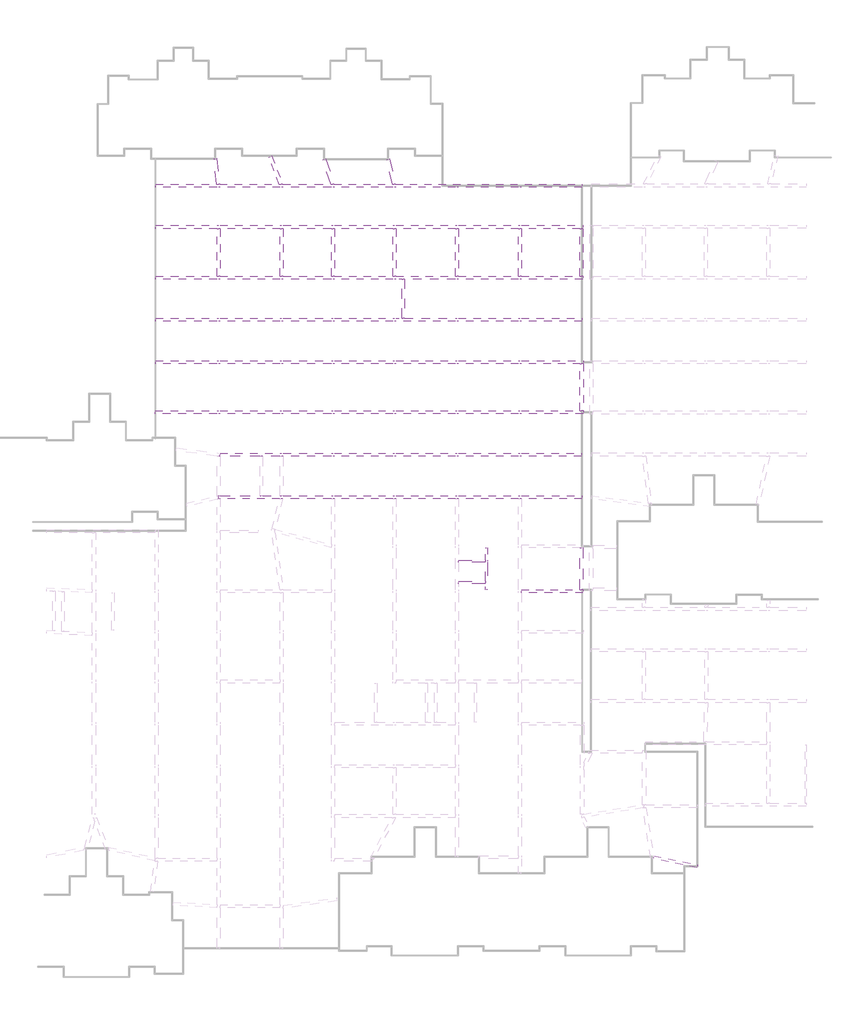
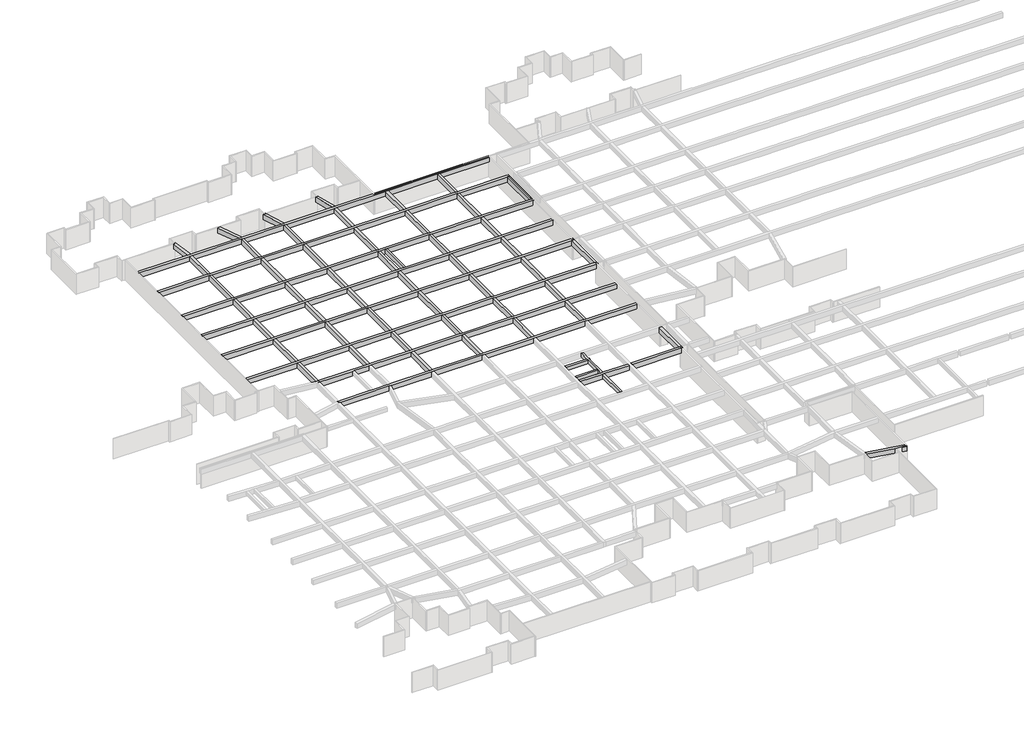
# One storey, part 11 of 16: 27 beams.
"""IFC4 building model written with IfcOpenShell, lengths in millimetres."""

from ifc_helpers import new_model, si_unit, frame, origin, place, context, project, spatial, polyline, outline, extrude, faceted_brep, element, save

model = new_model("IFC4")

# Units and contexts
model_context = context("Model", 3, world=origin())
ifc_project = project(units=[si_unit("LENGTHUNIT", "METRE", prefix="MILLI")], contexts=[model_context])

# Site, building, storey
site = spatial("IfcSite", under=ifc_project)
building = spatial("IfcBuilding", under=site)
storey = spatial("IfcBuildingStorey", under=building, Name="户型图", Elevation=0.0)

# Beams
placement = place(None, origin())
element("IfcBeam", 1, ObjectType="混凝土 - 矩形梁 : KL_beam", at=placement, inside=storey, context=model_context, shape_type="Brep", body=[
    faceted_brep([(255003.757676, -132325.7214763, 3300.0), (255003.757676, -132725.7214763, 3300.0), (255003.757676, -132725.7214763, 2500.0), (255003.757676, -132325.7214763, 2500.0), (200203.757676, -132325.7214763, 3300.0), (200203.757676, -132325.7214763, 2500.0), (200203.757676, -132725.7214763, 2500.0), (200203.757676, -132725.7214763, 3300.0), (231074.340029, -132325.7214763, 3300.0), (230661.8664477, -132325.7214763, 3300.0), (223163.2360526, -132325.7214763, 3300.0), (222740.8165445, -132325.7214763, 3300.0), (216536.3465944, -132325.7214763, 3300.0), (216107.8885969, -132325.7214763, 3300.0), (208493.8825468, -132325.7214763, 3300.0), (208090.4250487, -132325.7214763, 3300.0), (208121.0257524, -132725.7214763, 3300.0), (208521.0257524, -132725.7214763, 3300.0), (216198.8904026, -132725.7214763, 3300.0), (216598.8904026, -132725.7214763, 3300.0), (222798.8904026, -132725.7214763, 3300.0), (223198.8904026, -132725.7214763, 3300.0), (230718.438254, -132725.7214763, 3300.0), (231118.438254, -132725.7214763, 3300.0), (238718.438254, -132725.7214763, 3300.0), (239118.438254, -132725.7214763, 3300.0), (246818.438254, -132725.7214763, 3300.0), (247218.438254, -132725.7214763, 3300.0), (208121.0257524, -132725.7214763, 2500.0), (208521.0257524, -132725.7214763, 2500.0), (216198.8904026, -132725.7214763, 2500.0), (216598.8904026, -132725.7214763, 2500.0), (222798.8904026, -132725.7214763, 2500.0), (223198.8904026, -132725.7214763, 2500.0), (230718.438254, -132725.7214763, 2500.0), (231118.438254, -132725.7214763, 2500.0), (238718.438254, -132725.7214763, 2500.0), (239118.438254, -132725.7214763, 2500.0), (246818.438254, -132725.7214763, 2500.0), (247218.438254, -132725.7214763, 2500.0), (208090.4250487, -132325.7214763, 2500.0), (208493.8825468, -132325.7214763, 2500.0), (216107.8885969, -132325.7214763, 2500.0), (216536.3465944, -132325.7214763, 2500.0), (222740.8165445, -132325.7214763, 2500.0), (223163.2360526, -132325.7214763, 2500.0), (230661.8664477, -132325.7214763, 2500.0), (231074.340029, -132325.7214763, 2500.0)], [[[0, 1, 2, 3]], [[4, 5, 6, 7]], [[1, 0, 8, 9, 10, 11, 12, 13, 14, 15, 4, 7, 16, 17, 18, 19, 20, 21, 22, 23, 24, 25, 26, 27]], [[2, 1, 27, 26, 25, 24, 23, 22, 21, 20, 19, 18, 17, 16, 7, 6, 28, 29, 30, 31, 32, 33, 34, 35, 36, 37, 38, 39]], [[3, 2, 39, 38, 37, 36, 35, 34, 33, 32, 31, 30, 29, 28, 6, 5, 40, 41, 42, 43, 44, 45, 46, 47]], [[0, 3, 47, 46, 45, 44, 43, 42, 41, 40, 5, 4, 15, 14, 13, 12, 11, 10, 9, 8]]]),
])
element("IfcBeam", 2, ObjectType="混凝土 - 矩形梁 : KL_beam", at=placement, inside=storey, context=model_context, shape_type="SweptSolid", body=[
    extrude(outline(polyline([(207660.2352637, -129060.9134022), (208056.8073952, -129008.6587899), (208493.8825468, -132325.7214763), (208090.4250487, -132325.7214763), (207660.2352637, -129060.9134022)])), frame((0.0, 0.0, 2500.0), z_axis=(0.0, 0.0, 1.0), x_axis=(1.0, 0.0, 0.0)), (0.0, 0.0, 1.0), 800.0),
])
element("IfcBeam", 3, ObjectType="混凝土 - 矩形梁 : KL_beam", at=placement, inside=storey, context=model_context, shape_type="SweptSolid", body=[
    extrude(outline(polyline([(214772.1689398, -128846.0528041), (215145.6011104, -128702.7056243), (216536.3465944, -132325.7214763), (216107.8885969, -132325.7214763), (214772.1689398, -128846.0528041)])), frame((0.0, 0.0, 2500.0), z_axis=(0.0, 0.0, 1.0), x_axis=(1.0, 0.0, 0.0)), (0.0, 0.0, 1.0), 800.0),
])
element("IfcBeam", 4, ObjectType="混凝土 - 矩形梁 : KL_beam", at=placement, inside=storey, context=model_context, shape_type="SweptSolid", body=[
    extrude(outline(polyline([(221670.6359164, -129173.2052189), (222049.406302, -129044.6245246), (223163.2360526, -132325.7214763), (222740.8165445, -132325.7214763), (221670.6359164, -129173.2052189)])), frame((0.0, 0.0, 2500.0), z_axis=(0.0, 0.0, 1.0), x_axis=(1.0, 0.0, 0.0)), (0.0, 0.0, 1.0), 800.0),
])
element("IfcBeam", 5, ObjectType="混凝土 - 矩形梁 : KL_beam", at=placement, inside=storey, context=model_context, shape_type="SweptSolid", body=[
    extrude(outline(polyline([(229864.5673641, -129157.7515328), (230252.4709955, -129060.125856), (231074.340029, -132325.7214763), (230661.8664477, -132325.7214763), (229864.5673641, -129157.7515328)])), frame((0.0, 0.0, 2500.0), z_axis=(0.0, 0.0, 1.0), x_axis=(1.0, 0.0, 0.0)), (0.0, 0.0, 1.0), 800.0),
])
element("IfcBeam", 6, ObjectType="混凝土 - 矩形梁 : KL_beam", at=placement, inside=storey, context=model_context, shape_type="Brep", body=[
    faceted_brep([(200203.757676, -137625.7214763, 3300.0), (200203.757676, -137625.7214763, 2500.0), (200203.757676, -138025.7214763, 2500.0), (200203.757676, -138025.7214763, 3300.0), (208121.0257524, -138025.7214763, 3300.0), (208521.0257524, -138025.7214763, 3300.0), (216198.8904026, -138025.7214763, 3300.0), (216598.8904026, -138025.7214763, 3300.0), (222798.8904026, -138025.7214763, 3300.0), (223198.8904026, -138025.7214763, 3300.0), (230718.438254, -138025.7214763, 3300.0), (231118.438254, -138025.7214763, 3300.0), (238718.438254, -138025.7214763, 3300.0), (239118.438254, -138025.7214763, 3300.0), (246818.438254, -138025.7214763, 3300.0), (247218.438254, -138025.7214763, 3300.0), (254703.757676, -138025.7214763, 3300.0), (255103.757676, -138025.7214763, 3300.0), (255103.757676, -137625.7214763, 3300.0), (247218.438254, -137625.7214763, 3300.0), (246818.438254, -137625.7214763, 3300.0), (239118.438254, -137625.7214763, 3300.0), (238718.438254, -137625.7214763, 3300.0), (231118.438254, -137625.7214763, 3300.0), (230718.438254, -137625.7214763, 3300.0), (223198.8904026, -137625.7214763, 3300.0), (222798.8904026, -137625.7214763, 3300.0), (216598.8904026, -137625.7214763, 3300.0), (216198.8904026, -137625.7214763, 3300.0), (208521.0257524, -137625.7214763, 3300.0), (208121.0257524, -137625.7214763, 3300.0), (208121.0257524, -138025.7214763, 2500.0), (208521.0257524, -138025.7214763, 2500.0), (216198.8904026, -138025.7214763, 2500.0), (216598.8904026, -138025.7214763, 2500.0), (222798.8904026, -138025.7214763, 2500.0), (223198.8904026, -138025.7214763, 2500.0), (230718.438254, -138025.7214763, 2500.0), (231118.438254, -138025.7214763, 2500.0), (238718.438254, -138025.7214763, 2500.0), (239118.438254, -138025.7214763, 2500.0), (246818.438254, -138025.7214763, 2500.0), (247218.438254, -138025.7214763, 2500.0), (254703.757676, -138025.7214763, 2500.0), (255103.757676, -138025.7214763, 2500.0), (208121.0257524, -137625.7214763, 2500.0), (208521.0257524, -137625.7214763, 2500.0), (216198.8904026, -137625.7214763, 2500.0), (216598.8904026, -137625.7214763, 2500.0), (222798.8904026, -137625.7214763, 2500.0), (223198.8904026, -137625.7214763, 2500.0), (230718.438254, -137625.7214763, 2500.0), (231118.438254, -137625.7214763, 2500.0), (238718.438254, -137625.7214763, 2500.0), (239118.438254, -137625.7214763, 2500.0), (246818.438254, -137625.7214763, 2500.0), (247218.438254, -137625.7214763, 2500.0), (255103.757676, -137625.7214763, 2500.0)], [[[0, 1, 2, 3]], [[0, 3, 4, 5, 6, 7, 8, 9, 10, 11, 12, 13, 14, 15, 16, 17, 18, 19, 20, 21, 22, 23, 24, 25, 26, 27, 28, 29, 30]], [[3, 2, 31, 32, 33, 34, 35, 36, 37, 38, 39, 40, 41, 42, 43, 44, 17, 16, 15, 14, 13, 12, 11, 10, 9, 8, 7, 6, 5, 4]], [[2, 1, 45, 46, 47, 48, 49, 50, 51, 52, 53, 54, 55, 56, 57, 44, 43, 42, 41, 40, 39, 38, 37, 36, 35, 34, 33, 32, 31]], [[1, 0, 30, 29, 28, 27, 26, 25, 24, 23, 22, 21, 20, 19, 18, 57, 56, 55, 54, 53, 52, 51, 50, 49, 48, 47, 46, 45]], [[18, 17, 44, 57]]]),
])
element("IfcBeam", 7, ObjectType="混凝土 - 矩形梁 : KL_beam", at=placement, inside=storey, context=model_context, shape_type="Brep", body=[
    faceted_brep([(200203.757676, -144125.7214763, 3300.0), (200203.757676, -144125.7214763, 2500.0), (200203.757676, -144525.7214763, 2500.0), (200203.757676, -144525.7214763, 3300.0), (208121.0257524, -144525.7214763, 3300.0), (208521.0257524, -144525.7214763, 3300.0), (216198.8904026, -144525.7214763, 3300.0), (216598.8904026, -144525.7214763, 3300.0), (222798.8904026, -144525.7214763, 3300.0), (223198.8904026, -144525.7214763, 3300.0), (230718.438254, -144525.7214763, 3300.0), (231118.438254, -144525.7214763, 3300.0), (231868.438254, -144525.7214763, 3300.0), (232168.438254, -144525.7214763, 3300.0), (238718.438254, -144525.7214763, 3300.0), (239118.438254, -144525.7214763, 3300.0), (246818.438254, -144525.7214763, 3300.0), (247218.438254, -144525.7214763, 3300.0), (255103.757676, -144525.7214763, 3300.0), (255103.757676, -144125.7214763, 3300.0), (254703.757676, -144125.7214763, 3300.0), (247218.438254, -144125.7214763, 3300.0), (246818.438254, -144125.7214763, 3300.0), (239118.438254, -144125.7214763, 3300.0), (238718.438254, -144125.7214763, 3300.0), (231118.438254, -144125.7214763, 3300.0), (230718.438254, -144125.7214763, 3300.0), (223198.8904026, -144125.7214763, 3300.0), (222798.8904026, -144125.7214763, 3300.0), (216598.8904026, -144125.7214763, 3300.0), (216198.8904026, -144125.7214763, 3300.0), (208521.0257524, -144125.7214763, 3300.0), (208121.0257524, -144125.7214763, 3300.0), (208121.0257524, -144525.7214763, 2500.0), (208521.0257524, -144525.7214763, 2500.0), (216198.8904026, -144525.7214763, 2500.0), (216598.8904026, -144525.7214763, 2500.0), (222798.8904026, -144525.7214763, 2500.0), (223198.8904026, -144525.7214763, 2500.0), (230718.438254, -144525.7214763, 2500.0), (231118.438254, -144525.7214763, 2500.0), (238718.438254, -144525.7214763, 2500.0), (239118.438254, -144525.7214763, 2500.0), (246818.438254, -144525.7214763, 2500.0), (247218.438254, -144525.7214763, 2500.0), (255103.757676, -144525.7214763, 2500.0), (208121.0257524, -144125.7214763, 2500.0), (208521.0257524, -144125.7214763, 2500.0), (216198.8904026, -144125.7214763, 2500.0), (216598.8904026, -144125.7214763, 2500.0), (222798.8904026, -144125.7214763, 2500.0), (223198.8904026, -144125.7214763, 2500.0), (230718.438254, -144125.7214763, 2500.0), (231118.438254, -144125.7214763, 2500.0), (238718.438254, -144125.7214763, 2500.0), (239118.438254, -144125.7214763, 2500.0), (246818.438254, -144125.7214763, 2500.0), (247218.438254, -144125.7214763, 2500.0), (254703.757676, -144125.7214763, 2500.0), (255103.757676, -144125.7214763, 2500.0)], [[[0, 1, 2, 3]], [[0, 3, 4, 5, 6, 7, 8, 9, 10, 11, 12, 13, 14, 15, 16, 17, 18, 19, 20, 21, 22, 23, 24, 25, 26, 27, 28, 29, 30, 31, 32]], [[3, 2, 33, 34, 35, 36, 37, 38, 39, 40, 41, 42, 43, 44, 45, 18, 17, 16, 15, 14, 13, 12, 11, 10, 9, 8, 7, 6, 5, 4]], [[2, 1, 46, 47, 48, 49, 50, 51, 52, 53, 54, 55, 56, 57, 58, 59, 45, 44, 43, 42, 41, 40, 39, 38, 37, 36, 35, 34, 33]], [[1, 0, 32, 31, 30, 29, 28, 27, 26, 25, 24, 23, 22, 21, 20, 19, 59, 58, 57, 56, 55, 54, 53, 52, 51, 50, 49, 48, 47, 46]], [[19, 18, 45, 59]]]),
])
element("IfcBeam", 8, ObjectType="混凝土 - 矩形梁 : KL_beam", at=placement, inside=storey, context=model_context, shape_type="Brep", body=[
    faceted_brep([(255003.757676, -149525.7214763, 3300.0), (255003.757676, -149925.7214763, 3300.0), (255003.757676, -149925.7214763, 2500.0), (255003.757676, -149525.7214763, 2500.0), (200203.757676, -149525.7214763, 3300.0), (200203.757676, -149525.7214763, 2500.0), (200203.757676, -149925.7214763, 2500.0), (200203.757676, -149925.7214763, 3300.0), (247218.438254, -149525.7214763, 3300.0), (246818.438254, -149525.7214763, 3300.0), (239118.438254, -149525.7214763, 3300.0), (238718.438254, -149525.7214763, 3300.0), (232168.438254, -149525.7214763, 3300.0), (231868.438254, -149525.7214763, 3300.0), (231118.438254, -149525.7214763, 3300.0), (230718.438254, -149525.7214763, 3300.0), (223198.8904026, -149525.7214763, 3300.0), (222798.8904026, -149525.7214763, 3300.0), (216598.8904026, -149525.7214763, 3300.0), (216198.8904026, -149525.7214763, 3300.0), (208521.0257524, -149525.7214763, 3300.0), (208121.0257524, -149525.7214763, 3300.0), (208121.0257524, -149925.7214763, 3300.0), (208521.0257524, -149925.7214763, 3300.0), (216198.8904026, -149925.7214763, 3300.0), (216598.8904026, -149925.7214763, 3300.0), (222798.8904026, -149925.7214763, 3300.0), (223198.8904026, -149925.7214763, 3300.0), (230718.438254, -149925.7214763, 3300.0), (231118.438254, -149925.7214763, 3300.0), (238718.438254, -149925.7214763, 3300.0), (239118.438254, -149925.7214763, 3300.0), (246818.438254, -149925.7214763, 3300.0), (247218.438254, -149925.7214763, 3300.0), (208121.0257524, -149925.7214763, 2500.0), (208521.0257524, -149925.7214763, 2500.0), (216198.8904026, -149925.7214763, 2500.0), (216598.8904026, -149925.7214763, 2500.0), (222798.8904026, -149925.7214763, 2500.0), (223198.8904026, -149925.7214763, 2500.0), (230718.438254, -149925.7214763, 2500.0), (231118.438254, -149925.7214763, 2500.0), (238718.438254, -149925.7214763, 2500.0), (239118.438254, -149925.7214763, 2500.0), (246818.438254, -149925.7214763, 2500.0), (247218.438254, -149925.7214763, 2500.0), (208121.0257524, -149525.7214763, 2500.0), (208521.0257524, -149525.7214763, 2500.0), (216198.8904026, -149525.7214763, 2500.0), (216598.8904026, -149525.7214763, 2500.0), (222798.8904026, -149525.7214763, 2500.0), (223198.8904026, -149525.7214763, 2500.0), (230718.438254, -149525.7214763, 2500.0), (231118.438254, -149525.7214763, 2500.0), (238718.438254, -149525.7214763, 2500.0), (239118.438254, -149525.7214763, 2500.0), (246818.438254, -149525.7214763, 2500.0), (247218.438254, -149525.7214763, 2500.0)], [[[0, 1, 2, 3]], [[4, 5, 6, 7]], [[1, 0, 8, 9, 10, 11, 12, 13, 14, 15, 16, 17, 18, 19, 20, 21, 4, 7, 22, 23, 24, 25, 26, 27, 28, 29, 30, 31, 32, 33]], [[2, 1, 33, 32, 31, 30, 29, 28, 27, 26, 25, 24, 23, 22, 7, 6, 34, 35, 36, 37, 38, 39, 40, 41, 42, 43, 44, 45]], [[3, 2, 45, 44, 43, 42, 41, 40, 39, 38, 37, 36, 35, 34, 6, 5, 46, 47, 48, 49, 50, 51, 52, 53, 54, 55, 56, 57]], [[0, 3, 57, 56, 55, 54, 53, 52, 51, 50, 49, 48, 47, 46, 5, 4, 21, 20, 19, 18, 17, 16, 15, 14, 13, 12, 11, 10, 9, 8]]]),
])
element("IfcBeam", 9, ObjectType="混凝土 - 矩形梁 : KL_beam", at=placement, inside=storey, context=model_context, shape_type="Brep", body=[
    faceted_brep([(200203.757676, -154958.1403142, 3300.0), (200203.757676, -154958.1403142, 2500.0), (200203.757676, -155358.1403142, 2500.0), (200203.757676, -155358.1403142, 3300.0), (208121.0257524, -155358.1403142, 3300.0), (208521.0257524, -155358.1403142, 3300.0), (216198.8904026, -155358.1403142, 3300.0), (216598.8904026, -155358.1403142, 3300.0), (222798.8904026, -155358.1403142, 3300.0), (223198.8904026, -155358.1403142, 3300.0), (230718.438254, -155358.1403142, 3300.0), (231118.438254, -155358.1403142, 3300.0), (238718.438254, -155358.1403142, 3300.0), (239118.438254, -155358.1403142, 3300.0), (246818.438254, -155358.1403142, 3300.0), (247218.438254, -155358.1403142, 3300.0), (254753.757676, -155358.1403142, 3300.0), (255153.757676, -155358.1403142, 3300.0), (255153.757676, -154958.1403142, 3300.0), (247218.438254, -154958.1403142, 3300.0), (246818.438254, -154958.1403142, 3300.0), (239118.438254, -154958.1403142, 3300.0), (238718.438254, -154958.1403142, 3300.0), (231118.438254, -154958.1403142, 3300.0), (230718.438254, -154958.1403142, 3300.0), (223198.8904026, -154958.1403142, 3300.0), (222798.8904026, -154958.1403142, 3300.0), (216598.8904026, -154958.1403142, 3300.0), (216198.8904026, -154958.1403142, 3300.0), (208521.0257524, -154958.1403142, 3300.0), (208121.0257524, -154958.1403142, 3300.0), (208121.0257524, -155358.1403142, 2500.0), (208521.0257524, -155358.1403142, 2500.0), (216198.8904026, -155358.1403142, 2500.0), (216598.8904026, -155358.1403142, 2500.0), (222798.8904026, -155358.1403142, 2500.0), (223198.8904026, -155358.1403142, 2500.0), (230718.438254, -155358.1403142, 2500.0), (231118.438254, -155358.1403142, 2500.0), (238718.438254, -155358.1403142, 2500.0), (239118.438254, -155358.1403142, 2500.0), (246818.438254, -155358.1403142, 2500.0), (247218.438254, -155358.1403142, 2500.0), (254753.757676, -155358.1403142, 2500.0), (255153.757676, -155358.1403142, 2500.0), (208121.0257524, -154958.1403142, 2500.0), (208521.0257524, -154958.1403142, 2500.0), (216198.8904026, -154958.1403142, 2500.0), (216598.8904026, -154958.1403142, 2500.0), (222798.8904026, -154958.1403142, 2500.0), (223198.8904026, -154958.1403142, 2500.0), (230718.438254, -154958.1403142, 2500.0), (231118.438254, -154958.1403142, 2500.0), (238718.438254, -154958.1403142, 2500.0), (239118.438254, -154958.1403142, 2500.0), (246818.438254, -154958.1403142, 2500.0), (247218.438254, -154958.1403142, 2500.0), (255153.757676, -154958.1403142, 2500.0)], [[[0, 1, 2, 3]], [[0, 3, 4, 5, 6, 7, 8, 9, 10, 11, 12, 13, 14, 15, 16, 17, 18, 19, 20, 21, 22, 23, 24, 25, 26, 27, 28, 29, 30]], [[3, 2, 31, 32, 33, 34, 35, 36, 37, 38, 39, 40, 41, 42, 43, 44, 17, 16, 15, 14, 13, 12, 11, 10, 9, 8, 7, 6, 5, 4]], [[2, 1, 45, 46, 47, 48, 49, 50, 51, 52, 53, 54, 55, 56, 57, 44, 43, 42, 41, 40, 39, 38, 37, 36, 35, 34, 33, 32, 31]], [[1, 0, 30, 29, 28, 27, 26, 25, 24, 23, 22, 21, 20, 19, 18, 57, 56, 55, 54, 53, 52, 51, 50, 49, 48, 47, 46, 45]], [[18, 17, 44, 57]]]),
])
element("IfcBeam", 10, ObjectType="混凝土 - 矩形梁 : KL_beam", at=placement, inside=storey, context=model_context, shape_type="Brep", body=[
    faceted_brep([(200153.757676, -161405.1471774, 3300.0), (200153.757676, -161405.1471774, 2500.0), (200153.757676, -161805.1471774, 2500.0), (200153.757676, -161805.1471774, 3300.0), (208121.0257524, -161805.1471774, 3300.0), (208521.0257524, -161805.1471774, 3300.0), (216198.8904026, -161805.1471774, 3300.0), (216598.8904026, -161805.1471774, 3300.0), (222798.8904026, -161805.1471774, 3300.0), (223198.8904026, -161805.1471774, 3300.0), (230718.438254, -161805.1471774, 3300.0), (231118.438254, -161805.1471774, 3300.0), (238718.438254, -161805.1471774, 3300.0), (239118.438254, -161805.1471774, 3300.0), (246818.438254, -161805.1471774, 3300.0), (247218.438254, -161805.1471774, 3300.0), (255153.757676, -161805.1471774, 3300.0), (255153.757676, -161405.1471774, 3300.0), (254753.757676, -161405.1471774, 3300.0), (247218.438254, -161405.1471774, 3300.0), (246818.438254, -161405.1471774, 3300.0), (239118.438254, -161405.1471774, 3300.0), (238718.438254, -161405.1471774, 3300.0), (231118.438254, -161405.1471774, 3300.0), (230718.438254, -161405.1471774, 3300.0), (223198.8904026, -161405.1471774, 3300.0), (222798.8904026, -161405.1471774, 3300.0), (216598.8904026, -161405.1471774, 3300.0), (216198.8904026, -161405.1471774, 3300.0), (208521.0257524, -161405.1471774, 3300.0), (208121.0257524, -161405.1471774, 3300.0), (208121.0257524, -161805.1471774, 2500.0), (208521.0257524, -161805.1471774, 2500.0), (216198.8904026, -161805.1471774, 2500.0), (216598.8904026, -161805.1471774, 2500.0), (222798.8904026, -161805.1471774, 2500.0), (223198.8904026, -161805.1471774, 2500.0), (230718.438254, -161805.1471774, 2500.0), (231118.438254, -161805.1471774, 2500.0), (238718.438254, -161805.1471774, 2500.0), (239118.438254, -161805.1471774, 2500.0), (246818.438254, -161805.1471774, 2500.0), (247218.438254, -161805.1471774, 2500.0), (255153.757676, -161805.1471774, 2500.0), (208121.0257524, -161405.1471774, 2500.0), (208521.0257524, -161405.1471774, 2500.0), (216198.8904026, -161405.1471774, 2500.0), (216598.8904026, -161405.1471774, 2500.0), (222798.8904026, -161405.1471774, 2500.0), (223198.8904026, -161405.1471774, 2500.0), (230718.438254, -161405.1471774, 2500.0), (231118.438254, -161405.1471774, 2500.0), (238718.438254, -161405.1471774, 2500.0), (239118.438254, -161405.1471774, 2500.0), (246818.438254, -161405.1471774, 2500.0), (247218.438254, -161405.1471774, 2500.0), (254753.757676, -161405.1471774, 2500.0), (255153.757676, -161405.1471774, 2500.0)], [[[0, 1, 2, 3]], [[0, 3, 4, 5, 6, 7, 8, 9, 10, 11, 12, 13, 14, 15, 16, 17, 18, 19, 20, 21, 22, 23, 24, 25, 26, 27, 28, 29, 30]], [[3, 2, 31, 32, 33, 34, 35, 36, 37, 38, 39, 40, 41, 42, 43, 16, 15, 14, 13, 12, 11, 10, 9, 8, 7, 6, 5, 4]], [[2, 1, 44, 45, 46, 47, 48, 49, 50, 51, 52, 53, 54, 55, 56, 57, 43, 42, 41, 40, 39, 38, 37, 36, 35, 34, 33, 32, 31]], [[1, 0, 30, 29, 28, 27, 26, 25, 24, 23, 22, 21, 20, 19, 18, 17, 57, 56, 55, 54, 53, 52, 51, 50, 49, 48, 47, 46, 45, 44]], [[17, 16, 43, 57]]]),
])
element("IfcBeam", 11, ObjectType="混凝土 - 矩形梁 : KL_beam", at=placement, inside=storey, context=model_context, shape_type="Brep", body=[
    faceted_brep([(208521.0257524, -132725.7214763, 3300.0), (208121.0257524, -132725.7214763, 3300.0), (208121.0257524, -137625.7214763, 3300.0), (208521.0257524, -137625.7214763, 3300.0), (208521.0257524, -132725.7214763, 2500.0), (208521.0257524, -137625.7214763, 2500.0), (208121.0257524, -132725.7214763, 2500.0), (208121.0257524, -137625.7214763, 2500.0)], [[[0, 1, 2, 3]], [[4, 0, 3, 5]], [[6, 4, 5, 7]], [[1, 6, 7, 2]], [[1, 0, 4, 6]], [[3, 2, 7, 5]]]),
    faceted_brep([(208521.0257524, -166865.7269859, 3300.0), (208121.0257524, -166816.6131615, 3300.0), (208121.0257524, -166816.6131615, 2500.0), (208521.0257524, -166865.7269859, 2500.0), (208121.0257524, -161805.1471774, 3300.0), (208521.0257524, -161805.1471774, 3300.0), (208521.0257524, -161805.1471774, 2500.0), (208121.0257524, -161805.1471774, 2500.0), (208521.0257524, -166842.6720388, 3300.0), (208521.0257524, -166842.6720388, 2500.0)], [[[0, 1, 2, 3]], [[4, 5, 6, 7]], [[1, 0, 8, 5, 4]], [[0, 3, 9, 6, 5, 8]], [[3, 2, 7, 6, 9]], [[2, 1, 4, 7]]]),
    faceted_brep([(208121.0257524, -138025.7214763, 3300.0), (208521.0257524, -138025.7214763, 3300.0), (208521.0257524, -138025.7214763, 2500.0), (208121.0257524, -138025.7214763, 2500.0), (208121.0257524, -144125.7214763, 3300.0), (208521.0257524, -144125.7214763, 3300.0), (208521.0257524, -144125.7214763, 2500.0), (208121.0257524, -144125.7214763, 2500.0)], [[[0, 1, 2, 3]], [[1, 0, 4, 5]], [[2, 1, 5, 6]], [[3, 2, 6, 7]], [[0, 3, 7, 4]], [[5, 4, 7, 6]]]),
    faceted_brep([(208121.0257524, -144525.7214763, 3300.0), (208521.0257524, -144525.7214763, 3300.0), (208521.0257524, -144525.7214763, 2500.0), (208121.0257524, -144525.7214763, 2500.0), (208121.0257524, -149525.7214763, 3300.0), (208521.0257524, -149525.7214763, 3300.0), (208521.0257524, -149525.7214763, 2500.0), (208121.0257524, -149525.7214763, 2500.0)], [[[0, 1, 2, 3]], [[1, 0, 4, 5]], [[2, 1, 5, 6]], [[3, 2, 6, 7]], [[0, 3, 7, 4]], [[5, 4, 7, 6]]]),
    faceted_brep([(208121.0257524, -149925.7214763, 3300.0), (208521.0257524, -149925.7214763, 3300.0), (208521.0257524, -149925.7214763, 2500.0), (208121.0257524, -149925.7214763, 2500.0), (208121.0257524, -154958.1403142, 3300.0), (208521.0257524, -154958.1403142, 3300.0), (208521.0257524, -154958.1403142, 2500.0), (208121.0257524, -154958.1403142, 2500.0)], [[[0, 1, 2, 3]], [[1, 0, 4, 5]], [[2, 1, 5, 6]], [[3, 2, 6, 7]], [[0, 3, 7, 4]], [[5, 4, 7, 6]]]),
    faceted_brep([(208121.0257524, -155358.1403142, 3300.0), (208521.0257524, -155358.1403142, 3300.0), (208521.0257524, -155358.1403142, 2500.0), (208121.0257524, -155358.1403142, 2500.0), (208121.0257524, -161405.1471774, 3300.0), (208521.0257524, -161405.1471774, 3300.0), (208521.0257524, -161405.1471774, 2500.0), (208121.0257524, -161405.1471774, 2500.0)], [[[0, 1, 2, 3]], [[1, 0, 4, 5]], [[2, 1, 5, 6]], [[3, 2, 6, 7]], [[0, 3, 7, 4]], [[5, 4, 7, 6]]]),
])
element("IfcBeam", 12, ObjectType="混凝土 - 矩形梁 : KL_beam", at=placement, inside=storey, context=model_context, shape_type="SweptSolid", body=[
    extrude(outline(polyline([(216198.8904026, -161805.1471774), (216598.8904026, -161805.1471774), (216598.8904026, -166842.6720388), (216198.8904026, -166842.6720388), (216198.8904026, -161805.1471774)])), frame((0.0, 0.0, 2500.0), z_axis=(0.0, 0.0, 1.0), x_axis=(1.0, 0.0, 0.0)), (0.0, 0.0, 1.0), 800.0),
    extrude(outline(polyline([(216198.8904026, -132725.7214763), (216598.8904026, -132725.7214763), (216598.8904026, -137625.7214763), (216198.8904026, -137625.7214763), (216198.8904026, -132725.7214763)])), frame((0.0, 0.0, 2500.0), z_axis=(0.0, 0.0, 1.0), x_axis=(1.0, 0.0, 0.0)), (0.0, 0.0, 1.0), 800.0),
    extrude(outline(polyline([(216198.8904026, -138025.7214763), (216598.8904026, -138025.7214763), (216598.8904026, -144125.7214763), (216198.8904026, -144125.7214763), (216198.8904026, -138025.7214763)])), frame((0.0, 0.0, 2500.0), z_axis=(0.0, 0.0, 1.0), x_axis=(1.0, 0.0, 0.0)), (0.0, 0.0, 1.0), 800.0),
    extrude(outline(polyline([(216198.8904026, -144525.7214763), (216598.8904026, -144525.7214763), (216598.8904026, -149525.7214763), (216198.8904026, -149525.7214763), (216198.8904026, -144525.7214763)])), frame((0.0, 0.0, 2500.0), z_axis=(0.0, 0.0, 1.0), x_axis=(1.0, 0.0, 0.0)), (0.0, 0.0, 1.0), 800.0),
    extrude(outline(polyline([(216198.8904026, -149925.7214763), (216598.8904026, -149925.7214763), (216598.8904026, -154958.1403142), (216198.8904026, -154958.1403142), (216198.8904026, -149925.7214763)])), frame((0.0, 0.0, 2500.0), z_axis=(0.0, 0.0, 1.0), x_axis=(1.0, 0.0, 0.0)), (0.0, 0.0, 1.0), 800.0),
    extrude(outline(polyline([(216198.8904026, -155358.1403142), (216598.8904026, -155358.1403142), (216598.8904026, -161405.1471774), (216198.8904026, -161405.1471774), (216198.8904026, -155358.1403142)])), frame((0.0, 0.0, 2500.0), z_axis=(0.0, 0.0, 1.0), x_axis=(1.0, 0.0, 0.0)), (0.0, 0.0, 1.0), 800.0),
])
element("IfcBeam", 13, ObjectType="混凝土 - 矩形梁 : KL_beam", at=placement, inside=storey, context=model_context, shape_type="Brep", body=[
    faceted_brep([(254921.0257524, -166842.6720388, 3300.0), (254921.0257524, -167242.6720388, 3300.0), (254921.0257524, -167242.6720388, 2500.0), (254921.0257524, -166842.6720388, 2500.0), (247218.438254, -166842.6720388, 3300.0), (246818.438254, -166842.6720388, 3300.0), (239118.438254, -166842.6720388, 3300.0), (238718.438254, -166842.6720388, 3300.0), (231118.438254, -166842.6720388, 3300.0), (230718.438254, -166842.6720388, 3300.0), (223198.8904026, -166842.6720388, 3300.0), (222798.8904026, -166842.6720388, 3300.0), (216598.8904026, -166842.6720388, 3300.0), (216198.8904026, -166842.6720388, 3300.0), (208521.0257524, -166842.6720388, 3300.0), (208521.0257524, -166865.7269859, 3300.0), (208474.7427196, -167242.6720388, 3300.0), (208521.0257524, -167242.6720388, 3300.0), (213648.8904026, -167242.6720388, 3300.0), (213948.8904026, -167242.6720388, 3300.0), (216198.8904026, -167242.6720388, 3300.0), (216598.8904026, -167242.6720388, 3300.0), (222798.8904026, -167242.6720388, 3300.0), (223198.8904026, -167242.6720388, 3300.0), (230718.438254, -167242.6720388, 3300.0), (231118.438254, -167242.6720388, 3300.0), (238718.438254, -167242.6720388, 3300.0), (239118.438254, -167242.6720388, 3300.0), (246818.438254, -167242.6720388, 3300.0), (247218.438254, -167242.6720388, 3300.0), (208474.7427196, -167242.6720388, 2500.0), (208521.0257524, -167242.6720388, 2500.0), (216198.8904026, -167242.6720388, 2500.0), (216598.8904026, -167242.6720388, 2500.0), (222798.8904026, -167242.6720388, 2500.0), (223198.8904026, -167242.6720388, 2500.0), (230718.438254, -167242.6720388, 2500.0), (231118.438254, -167242.6720388, 2500.0), (238718.438254, -167242.6720388, 2500.0), (239118.438254, -167242.6720388, 2500.0), (246818.438254, -167242.6720388, 2500.0), (247218.438254, -167242.6720388, 2500.0), (208521.0257524, -166865.7269859, 2500.0), (208521.0257524, -166842.6720388, 2500.0), (216198.8904026, -166842.6720388, 2500.0), (216598.8904026, -166842.6720388, 2500.0), (222798.8904026, -166842.6720388, 2500.0), (223198.8904026, -166842.6720388, 2500.0), (230718.438254, -166842.6720388, 2500.0), (231118.438254, -166842.6720388, 2500.0), (238718.438254, -166842.6720388, 2500.0), (239118.438254, -166842.6720388, 2500.0), (246818.438254, -166842.6720388, 2500.0), (247218.438254, -166842.6720388, 2500.0)], [[[0, 1, 2, 3]], [[1, 0, 4, 5, 6, 7, 8, 9, 10, 11, 12, 13, 14, 15, 16, 17, 18, 19, 20, 21, 22, 23, 24, 25, 26, 27, 28, 29]], [[2, 1, 29, 28, 27, 26, 25, 24, 23, 22, 21, 20, 19, 18, 17, 16, 30, 31, 32, 33, 34, 35, 36, 37, 38, 39, 40, 41]], [[3, 2, 41, 40, 39, 38, 37, 36, 35, 34, 33, 32, 31, 30, 42, 43, 44, 45, 46, 47, 48, 49, 50, 51, 52, 53]], [[0, 3, 53, 52, 51, 50, 49, 48, 47, 46, 45, 44, 43, 14, 13, 12, 11, 10, 9, 8, 7, 6, 5, 4]], [[16, 15, 42, 30]], [[15, 14, 43, 42]]]),
    faceted_brep([(208121.0257524, -167242.6720388, 2500.0), (208121.0257524, -167242.6720388, 3300.0), (208121.0257524, -167219.6170917, 3300.0), (208121.0257524, -167219.6170917, 2500.0), (208308.7932284, -167242.6720388, 3300.0), (208308.7932284, -167242.6720388, 2500.0)], [[[0, 1, 2, 3]], [[2, 4, 5, 3]], [[1, 4, 2]], [[1, 0, 5, 4]], [[5, 0, 3]]]),
])
element("IfcBeam", 14, ObjectType="混凝土 - 矩形梁 : KL_beam", at=placement, inside=storey, context=model_context, shape_type="Brep", body=[
    faceted_brep([(254997.6165823, -172334.8916503, 3300.0), (254997.6165823, -172734.8916503, 3300.0), (254997.6165823, -172734.8916503, 2500.0), (254997.6165823, -172334.8916503, 2500.0), (247218.438254, -172334.8916503, 3300.0), (246818.438254, -172334.8916503, 3300.0), (239118.438254, -172334.8916503, 3300.0), (238718.438254, -172334.8916503, 3300.0), (231118.438254, -172334.8916503, 3300.0), (230718.438254, -172334.8916503, 3300.0), (223198.8904026, -172334.8916503, 3300.0), (222798.8904026, -172334.8916503, 3300.0), (216598.8904026, -172334.8916503, 3300.0), (216198.8904026, -172334.8916503, 3300.0), (213948.8904026, -172334.8916503, 3300.0), (213648.8904026, -172334.8916503, 3300.0), (208521.0257524, -172334.8916503, 3300.0), (208274.8294606, -172334.8916503, 3300.0), (208320.403704, -172734.8916503, 3300.0), (208521.0257524, -172734.8916503, 3300.0), (216141.6200419, -172734.8916503, 3300.0), (216554.3688646, -172734.8916503, 3300.0), (222798.8904026, -172734.8916503, 3300.0), (223198.8904026, -172734.8916503, 3300.0), (230718.438254, -172734.8916503, 3300.0), (231118.438254, -172734.8916503, 3300.0), (238718.438254, -172734.8916503, 3300.0), (239118.438254, -172734.8916503, 3300.0), (246818.438254, -172734.8916503, 3300.0), (247218.438254, -172734.8916503, 3300.0), (208320.403704, -172734.8916503, 2500.0), (208521.0257524, -172734.8916503, 2500.0), (216141.6200419, -172734.8916503, 2500.0), (216554.3688646, -172734.8916503, 2500.0), (222798.8904026, -172734.8916503, 2500.0), (223198.8904026, -172734.8916503, 2500.0), (230718.438254, -172734.8916503, 2500.0), (231118.438254, -172734.8916503, 2500.0), (238718.438254, -172734.8916503, 2500.0), (239118.438254, -172734.8916503, 2500.0), (246818.438254, -172734.8916503, 2500.0), (247218.438254, -172734.8916503, 2500.0), (208274.8294606, -172334.8916503, 2500.0), (208521.0257524, -172334.8916503, 2500.0), (216198.8904026, -172334.8916503, 2500.0), (216598.8904026, -172334.8916503, 2500.0), (222798.8904026, -172334.8916503, 2500.0), (223198.8904026, -172334.8916503, 2500.0), (230718.438254, -172334.8916503, 2500.0), (231118.438254, -172334.8916503, 2500.0), (238718.438254, -172334.8916503, 2500.0), (239118.438254, -172334.8916503, 2500.0), (246818.438254, -172334.8916503, 2500.0), (247218.438254, -172334.8916503, 2500.0)], [[[0, 1, 2, 3]], [[1, 0, 4, 5, 6, 7, 8, 9, 10, 11, 12, 13, 14, 15, 16, 17, 18, 19, 20, 21, 22, 23, 24, 25, 26, 27, 28, 29]], [[2, 1, 29, 28, 27, 26, 25, 24, 23, 22, 21, 20, 19, 18, 30, 31, 32, 33, 34, 35, 36, 37, 38, 39, 40, 41]], [[3, 2, 41, 40, 39, 38, 37, 36, 35, 34, 33, 32, 31, 30, 42, 43, 44, 45, 46, 47, 48, 49, 50, 51, 52, 53]], [[0, 3, 53, 52, 51, 50, 49, 48, 47, 46, 45, 44, 43, 42, 17, 16, 15, 14, 13, 12, 11, 10, 9, 8, 7, 6, 5, 4]], [[17, 42, 30, 18]]]),
])
element("IfcBeam", 15, ObjectType="混凝土 - 矩形梁 : KL_beam", at=placement, inside=storey, context=model_context, shape_type="SweptSolid", body=[
    extrude(outline(polyline([(223198.8904026, -172334.8916503), (222798.8904026, -172334.8916503), (222798.8904026, -167242.6720388), (223198.8904026, -167242.6720388), (223198.8904026, -172334.8916503)])), frame((0.0, 0.0, 2500.0), z_axis=(0.0, 0.0, 1.0), x_axis=(1.0, 0.0, 0.0)), (0.0, 0.0, 1.0), 800.0),
    extrude(outline(polyline([(222798.8904026, -132725.7214763), (223198.8904026, -132725.7214763), (223198.8904026, -137625.7214763), (222798.8904026, -137625.7214763), (222798.8904026, -132725.7214763)])), frame((0.0, 0.0, 2500.0), z_axis=(0.0, 0.0, 1.0), x_axis=(1.0, 0.0, 0.0)), (0.0, 0.0, 1.0), 800.0),
    extrude(outline(polyline([(222798.8904026, -138025.7214763), (223198.8904026, -138025.7214763), (223198.8904026, -144125.7214763), (222798.8904026, -144125.7214763), (222798.8904026, -138025.7214763)])), frame((0.0, 0.0, 2500.0), z_axis=(0.0, 0.0, 1.0), x_axis=(1.0, 0.0, 0.0)), (0.0, 0.0, 1.0), 800.0),
    extrude(outline(polyline([(222798.8904026, -144525.7214763), (223198.8904026, -144525.7214763), (223198.8904026, -149525.7214763), (222798.8904026, -149525.7214763), (222798.8904026, -144525.7214763)])), frame((0.0, 0.0, 2500.0), z_axis=(0.0, 0.0, 1.0), x_axis=(1.0, 0.0, 0.0)), (0.0, 0.0, 1.0), 800.0),
    extrude(outline(polyline([(222798.8904026, -149925.7214763), (223198.8904026, -149925.7214763), (223198.8904026, -154958.1403142), (222798.8904026, -154958.1403142), (222798.8904026, -149925.7214763)])), frame((0.0, 0.0, 2500.0), z_axis=(0.0, 0.0, 1.0), x_axis=(1.0, 0.0, 0.0)), (0.0, 0.0, 1.0), 800.0),
    extrude(outline(polyline([(222798.8904026, -155358.1403142), (223198.8904026, -155358.1403142), (223198.8904026, -161405.1471774), (222798.8904026, -161405.1471774), (222798.8904026, -155358.1403142)])), frame((0.0, 0.0, 2500.0), z_axis=(0.0, 0.0, 1.0), x_axis=(1.0, 0.0, 0.0)), (0.0, 0.0, 1.0), 800.0),
    extrude(outline(polyline([(222798.8904026, -161805.1471774), (223198.8904026, -161805.1471774), (223198.8904026, -166842.6720388), (222798.8904026, -166842.6720388), (222798.8904026, -161805.1471774)])), frame((0.0, 0.0, 2500.0), z_axis=(0.0, 0.0, 1.0), x_axis=(1.0, 0.0, 0.0)), (0.0, 0.0, 1.0), 800.0),
])
element("IfcBeam", 16, ObjectType="混凝土 - 矩形梁 : KL_beam", at=placement, inside=storey, context=model_context, shape_type="SweptSolid", body=[
    extrude(outline(polyline([(230718.438254, -132725.7214763), (231118.438254, -132725.7214763), (231118.438254, -137625.7214763), (230718.438254, -137625.7214763), (230718.438254, -132725.7214763)])), frame((0.0, 0.0, 2500.0), z_axis=(0.0, 0.0, 1.0), x_axis=(1.0, 0.0, 0.0)), (0.0, 0.0, 1.0), 800.0),
    extrude(outline(polyline([(231118.438254, -172334.8916503), (230718.438254, -172334.8916503), (230718.438254, -167242.6720388), (231118.438254, -167242.6720388), (231118.438254, -172334.8916503)])), frame((0.0, 0.0, 2500.0), z_axis=(0.0, 0.0, 1.0), x_axis=(1.0, 0.0, 0.0)), (0.0, 0.0, 1.0), 800.0),
    extrude(outline(polyline([(230718.438254, -138025.7214763), (231118.438254, -138025.7214763), (231118.438254, -144125.7214763), (230718.438254, -144125.7214763), (230718.438254, -138025.7214763)])), frame((0.0, 0.0, 2500.0), z_axis=(0.0, 0.0, 1.0), x_axis=(1.0, 0.0, 0.0)), (0.0, 0.0, 1.0), 800.0),
    extrude(outline(polyline([(230718.438254, -144525.7214763), (231118.438254, -144525.7214763), (231118.438254, -149525.7214763), (230718.438254, -149525.7214763), (230718.438254, -144525.7214763)])), frame((0.0, 0.0, 2500.0), z_axis=(0.0, 0.0, 1.0), x_axis=(1.0, 0.0, 0.0)), (0.0, 0.0, 1.0), 800.0),
    extrude(outline(polyline([(230718.438254, -149925.7214763), (231118.438254, -149925.7214763), (231118.438254, -154958.1403142), (230718.438254, -154958.1403142), (230718.438254, -149925.7214763)])), frame((0.0, 0.0, 2500.0), z_axis=(0.0, 0.0, 1.0), x_axis=(1.0, 0.0, 0.0)), (0.0, 0.0, 1.0), 800.0),
    extrude(outline(polyline([(230718.438254, -155358.1403142), (231118.438254, -155358.1403142), (231118.438254, -161405.1471774), (230718.438254, -161405.1471774), (230718.438254, -155358.1403142)])), frame((0.0, 0.0, 2500.0), z_axis=(0.0, 0.0, 1.0), x_axis=(1.0, 0.0, 0.0)), (0.0, 0.0, 1.0), 800.0),
    extrude(outline(polyline([(230718.438254, -161805.1471774), (231118.438254, -161805.1471774), (231118.438254, -166842.6720388), (230718.438254, -166842.6720388), (230718.438254, -161805.1471774)])), frame((0.0, 0.0, 2500.0), z_axis=(0.0, 0.0, 1.0), x_axis=(1.0, 0.0, 0.0)), (0.0, 0.0, 1.0), 800.0),
])
element("IfcBeam", 17, ObjectType="混凝土 - 矩形梁 : KL_beam", at=placement, inside=storey, context=model_context, shape_type="SweptSolid", body=[
    extrude(outline(polyline([(239118.438254, -172334.8916503), (238718.438254, -172334.8916503), (238718.438254, -167242.6720388), (239118.438254, -167242.6720388), (239118.438254, -172334.8916503)])), frame((0.0, 0.0, 2500.0), z_axis=(0.0, 0.0, 1.0), x_axis=(1.0, 0.0, 0.0)), (0.0, 0.0, 1.0), 800.0),
    extrude(outline(polyline([(238718.438254, -132725.7214763), (239118.438254, -132725.7214763), (239118.438254, -137625.7214763), (238718.438254, -137625.7214763), (238718.438254, -132725.7214763)])), frame((0.0, 0.0, 2500.0), z_axis=(0.0, 0.0, 1.0), x_axis=(1.0, 0.0, 0.0)), (0.0, 0.0, 1.0), 800.0),
    extrude(outline(polyline([(238718.438254, -138025.7214763), (239118.438254, -138025.7214763), (239118.438254, -144125.7214763), (238718.438254, -144125.7214763), (238718.438254, -138025.7214763)])), frame((0.0, 0.0, 2500.0), z_axis=(0.0, 0.0, 1.0), x_axis=(1.0, 0.0, 0.0)), (0.0, 0.0, 1.0), 800.0),
    extrude(outline(polyline([(238718.438254, -144525.7214763), (239118.438254, -144525.7214763), (239118.438254, -149525.7214763), (238718.438254, -149525.7214763), (238718.438254, -144525.7214763)])), frame((0.0, 0.0, 2500.0), z_axis=(0.0, 0.0, 1.0), x_axis=(1.0, 0.0, 0.0)), (0.0, 0.0, 1.0), 800.0),
    extrude(outline(polyline([(238718.438254, -149925.7214763), (239118.438254, -149925.7214763), (239118.438254, -154958.1403142), (238718.438254, -154958.1403142), (238718.438254, -149925.7214763)])), frame((0.0, 0.0, 2500.0), z_axis=(0.0, 0.0, 1.0), x_axis=(1.0, 0.0, 0.0)), (0.0, 0.0, 1.0), 800.0),
    extrude(outline(polyline([(238718.438254, -155358.1403142), (239118.438254, -155358.1403142), (239118.438254, -161405.1471774), (238718.438254, -161405.1471774), (238718.438254, -155358.1403142)])), frame((0.0, 0.0, 2500.0), z_axis=(0.0, 0.0, 1.0), x_axis=(1.0, 0.0, 0.0)), (0.0, 0.0, 1.0), 800.0),
    extrude(outline(polyline([(238718.438254, -161805.1471774), (239118.438254, -161805.1471774), (239118.438254, -166842.6720388), (238718.438254, -166842.6720388), (238718.438254, -161805.1471774)])), frame((0.0, 0.0, 2500.0), z_axis=(0.0, 0.0, 1.0), x_axis=(1.0, 0.0, 0.0)), (0.0, 0.0, 1.0), 800.0),
])
element("IfcBeam", 18, ObjectType="混凝土 - 矩形梁 : KL_beam", at=placement, inside=storey, context=model_context, shape_type="SweptSolid", body=[
    extrude(outline(polyline([(246818.438254, -132725.7214763), (247218.438254, -132725.7214763), (247218.438254, -137625.7214763), (246818.438254, -137625.7214763), (246818.438254, -132725.7214763)])), frame((0.0, 0.0, 2500.0), z_axis=(0.0, 0.0, 1.0), x_axis=(1.0, 0.0, 0.0)), (0.0, 0.0, 1.0), 800.0),
    extrude(outline(polyline([(247218.438254, -172334.8916503), (246818.438254, -172334.8916503), (246818.438254, -167242.6720388), (247218.438254, -167242.6720388), (247218.438254, -172334.8916503)])), frame((0.0, 0.0, 2500.0), z_axis=(0.0, 0.0, 1.0), x_axis=(1.0, 0.0, 0.0)), (0.0, 0.0, 1.0), 800.0),
    extrude(outline(polyline([(246818.438254, -138025.7214763), (247218.438254, -138025.7214763), (247218.438254, -144125.7214763), (246818.438254, -144125.7214763), (246818.438254, -138025.7214763)])), frame((0.0, 0.0, 2500.0), z_axis=(0.0, 0.0, 1.0), x_axis=(1.0, 0.0, 0.0)), (0.0, 0.0, 1.0), 800.0),
    extrude(outline(polyline([(246818.438254, -144525.7214763), (247218.438254, -144525.7214763), (247218.438254, -149525.7214763), (246818.438254, -149525.7214763), (246818.438254, -144525.7214763)])), frame((0.0, 0.0, 2500.0), z_axis=(0.0, 0.0, 1.0), x_axis=(1.0, 0.0, 0.0)), (0.0, 0.0, 1.0), 800.0),
    extrude(outline(polyline([(246818.438254, -149925.7214763), (247218.438254, -149925.7214763), (247218.438254, -154958.1403142), (246818.438254, -154958.1403142), (246818.438254, -149925.7214763)])), frame((0.0, 0.0, 2500.0), z_axis=(0.0, 0.0, 1.0), x_axis=(1.0, 0.0, 0.0)), (0.0, 0.0, 1.0), 800.0),
    extrude(outline(polyline([(246818.438254, -155358.1403142), (247218.438254, -155358.1403142), (247218.438254, -161405.1471774), (246818.438254, -161405.1471774), (246818.438254, -155358.1403142)])), frame((0.0, 0.0, 2500.0), z_axis=(0.0, 0.0, 1.0), x_axis=(1.0, 0.0, 0.0)), (0.0, 0.0, 1.0), 800.0),
    extrude(outline(polyline([(246818.438254, -161805.1471774), (247218.438254, -161805.1471774), (247218.438254, -166842.6720388), (246818.438254, -166842.6720388), (246818.438254, -161805.1471774)])), frame((0.0, 0.0, 2500.0), z_axis=(0.0, 0.0, 1.0), x_axis=(1.0, 0.0, 0.0)), (0.0, 0.0, 1.0), 800.0),
])
element("IfcBeam", 19, ObjectType="混凝土 - 矩形梁 : KL_beam", at=placement, inside=storey, context=model_context, shape_type="Brep", body=[
    faceted_brep([(239118.438254, -184365.1471774, 3300.0), (239118.438254, -184765.1471774, 3300.0), (242568.438254, -184765.1471774, 3300.0), (242868.438254, -184765.1471774, 3300.0), (246818.438254, -184765.1471774, 3300.0), (246818.438254, -184365.1471774, 3300.0), (242868.438254, -184365.1471774, 3300.0), (242568.438254, -184365.1471774, 3300.0), (239118.438254, -184765.1471774, 2500.0), (246818.438254, -184765.1471774, 2500.0), (239118.438254, -184365.1471774, 2500.0), (246818.438254, -184365.1471774, 2500.0)], [[[0, 1, 2, 3, 4, 5, 6, 7]], [[1, 8, 9, 4, 3, 2]], [[8, 10, 11, 9]], [[10, 0, 7, 6, 5, 11]], [[1, 0, 10, 8]], [[5, 4, 9, 11]]]),
    faceted_brep([(247218.438254, -184765.1471774, 3300.0), (247218.438254, -184365.1471774, 3300.0), (247218.438254, -184365.1471774, 2500.0), (247218.438254, -184765.1471774, 2500.0), (255118.438254, -184765.1471774, 3300.0), (255118.438254, -184365.1471774, 3300.0), (254718.438254, -184365.1471774, 3300.0), (255118.438254, -184765.1471774, 2500.0), (255118.438254, -184365.1471774, 2500.0), (254718.438254, -184365.1471774, 2500.0)], [[[0, 1, 2, 3]], [[4, 5, 6, 1, 0]], [[7, 4, 0, 3]], [[8, 7, 3, 2, 9]], [[5, 8, 9, 2, 1, 6]], [[5, 4, 7, 8]]]),
])
element("IfcBeam", 20, ObjectType="混凝土 - 矩形梁 : KL_beam", at=placement, inside=storey, context=model_context, shape_type="SweptSolid", body=[
    extrude(outline(polyline([(255118.438254, -184365.1471774), (254718.438254, -184365.1471774), (254718.438254, -179026.0461868), (255118.438254, -179026.0461868), (255118.438254, -184365.1471774)])), frame((0.0, 0.0, 2500.0), z_axis=(0.0, 0.0, 1.0), x_axis=(1.0, 0.0, 0.0)), (0.0, 0.0, 1.0), 800.0),
])
element("IfcBeam", 21, ObjectType="混凝土 - 矩形梁 : KL_beam", at=placement, inside=storey, context=model_context, shape_type="SweptSolid", body=[
    extrude(outline(polyline([(254753.757676, -155358.1403142), (255153.757676, -155358.1403142), (255153.757676, -161405.1471774), (254753.757676, -161405.1471774), (254753.757676, -155358.1403142)])), frame((0.0, 0.0, 2500.0), z_axis=(0.0, 0.0, 1.0), x_axis=(1.0, 0.0, 0.0)), (0.0, 0.0, 1.0), 800.0),
])
element("IfcBeam", 22, ObjectType="混凝土 - 矩形梁 : KL_beam", at=placement, inside=storey, context=model_context, shape_type="SweptSolid", body=[
    extrude(outline(polyline([(254703.757676, -138025.7214763), (255103.757676, -138025.7214763), (255103.757676, -144125.7214763), (254703.757676, -144125.7214763), (254703.757676, -138025.7214763)])), frame((0.0, 0.0, 2500.0), z_axis=(0.0, 0.0, 1.0), x_axis=(1.0, 0.0, 0.0)), (0.0, 0.0, 1.0), 800.0),
])
element("IfcBeam", 23, ObjectType="混凝土 - 矩形梁 : KL_beam", at=placement, inside=storey, context=model_context, shape_type="SweptSolid", body=[
    extrude(outline(polyline([(269843.555186, -219677.7535672), (269763.0321845, -220069.5648052), (264249.6949513, -218936.4925009), (264182.8409764, -218514.3931156), (269843.555186, -219677.7535672)])), frame((0.0, 0.0, 2500.0), z_axis=(0.0, 0.0, 1.0), x_axis=(1.0, 0.0, 0.0)), (0.0, 0.0, 1.0), 800.0),
])
element("IfcBeam", 24, ObjectType="混凝土 - 矩形梁 : L_beam", at=placement, inside=storey, context=model_context, shape_type="SweptSolid", body=[
    extrude(outline(polyline([(231868.438254, -144525.7214763), (232168.438254, -144525.7214763), (232168.438254, -149525.7214763), (231868.438254, -149525.7214763), (231868.438254, -144525.7214763)])), frame((0.0, 0.0, 2700.0), z_axis=(0.0, 0.0, 1.0), x_axis=(1.0, 0.0, 0.0)), (0.0, 0.0, 1.0), 600.0),
])
element("IfcBeam", 25, ObjectType="混凝土 - 矩形梁 : L_beam", at=placement, inside=storey, context=model_context, shape_type="Brep", body=[
    faceted_brep([(242568.438254, -189565.1471774, 3300.0), (242868.438254, -189565.1471774, 3300.0), (242868.438254, -184765.1471774, 3300.0), (242568.438254, -184765.1471774, 3300.0), (242868.438254, -189565.1471774, 2700.0), (242868.438254, -184765.1471774, 2700.0), (242568.438254, -189565.1471774, 2700.0), (242568.438254, -184765.1471774, 2700.0)], [[[0, 1, 2, 3]], [[1, 4, 5, 2]], [[4, 6, 7, 5]], [[6, 0, 3, 7]], [[1, 0, 6, 4]], [[3, 2, 5, 7]]]),
    faceted_brep([(242568.438254, -179026.0461868, 3300.0), (242868.438254, -179026.0461868, 3300.0), (242868.438254, -179026.0461868, 2700.0), (242568.438254, -179026.0461868, 2700.0), (242868.438254, -184365.1471774, 3300.0), (242568.438254, -184365.1471774, 3300.0), (242568.438254, -184365.1471774, 2700.0), (242868.438254, -184365.1471774, 2700.0), (242568.438254, -180576.0461868, 3300.0), (242568.438254, -180876.0461868, 3300.0), (242568.438254, -183315.1471774, 3300.0), (242568.438254, -183615.1471774, 3300.0), (242868.438254, -180876.0461868, 3300.0), (242868.438254, -180576.0461868, 3300.0), (242868.438254, -180876.0461868, 2700.0), (242868.438254, -180576.0461868, 2700.0), (242568.438254, -183615.1471774, 2700.0), (242568.438254, -183315.1471774, 2700.0), (242568.438254, -180876.0461868, 2700.0), (242568.438254, -180576.0461868, 2700.0)], [[[0, 1, 2, 3]], [[4, 5, 6, 7]], [[1, 0, 8, 9, 10, 11, 5, 4, 12, 13]], [[2, 1, 13, 12, 4, 7, 14, 15]], [[3, 2, 15, 14, 7, 6, 16, 17, 18, 19]], [[0, 3, 19, 18, 17, 16, 6, 5, 11, 10, 9, 8]]]),
])
element("IfcBeam", 26, ObjectType="混凝土 - 矩形梁 : L_beam", at=placement, inside=storey, context=model_context, shape_type="SweptSolid", body=[
    extrude(outline(polyline([(242918.438254, -180576.0461868), (242918.438254, -180876.0461868), (242868.438254, -180876.0461868), (242868.438254, -180576.0461868), (242918.438254, -180576.0461868)])), frame((0.0, 0.0, 2700.0), z_axis=(0.0, 0.0, 1.0), x_axis=(1.0, 0.0, 0.0)), (0.0, 0.0, 1.0), 600.0),
    extrude(outline(polyline([(239118.438254, -180876.0461868), (239118.438254, -180576.0461868), (242568.438254, -180576.0461868), (242568.438254, -180876.0461868), (239118.438254, -180876.0461868)])), frame((0.0, 0.0, 2700.0), z_axis=(0.0, 0.0, 1.0), x_axis=(1.0, 0.0, 0.0)), (0.0, 0.0, 1.0), 600.0),
])
element("IfcBeam", 27, ObjectType="混凝土 - 矩形梁 : L_beam", at=placement, inside=storey, context=model_context, shape_type="SweptSolid", body=[
    extrude(outline(polyline([(239118.438254, -183615.1471774), (239118.438254, -183315.1471774), (242568.438254, -183315.1471774), (242568.438254, -183615.1471774), (239118.438254, -183615.1471774)])), frame((0.0, 0.0, 2700.0), z_axis=(0.0, 0.0, 1.0), x_axis=(1.0, 0.0, 0.0)), (0.0, 0.0, 1.0), 600.0),
])

save(model, "model.ifc")

# Revit data of these elements
# Type "混凝土 - 矩形梁 : KL_beam"
#   Length [instance default] = 1524 mm
#   b = 400 mm
#   h = 800 mm
#   Structural Material [instance default] = 混凝土 - 现场浇注混凝土
#   Assembly Code = ""
# Type "混凝土 - 矩形梁 : L_beam"
#   Length [instance default] = 1524 mm
#   b = 300 mm
#   h = 600 mm
#   Structural Material [instance default] = none
#   Assembly Code = ""
# Elements 1, 2, 3, 4, 5, 6, 7, 8, 9, 10, 11, 12, 13, 14, 15, 16, 17, 18, 19, 20, 21, 22, 23 (IfcBeam, "混凝土 - 矩形梁 : KL_beam")
#   Comments = ""
#   Structural Material = none
#   Phase Created = 新构造
# Elements 24, 25, 26, 27 (IfcBeam, "混凝土 - 矩形梁 : L_beam")
#   Comments = ""
#   Structural Material = none
#   Phase Created = 新构造
# Materials
#   "混凝土 - 现场浇注混凝土": class "混凝土", colour RGB 192 192 192, transparency 0
